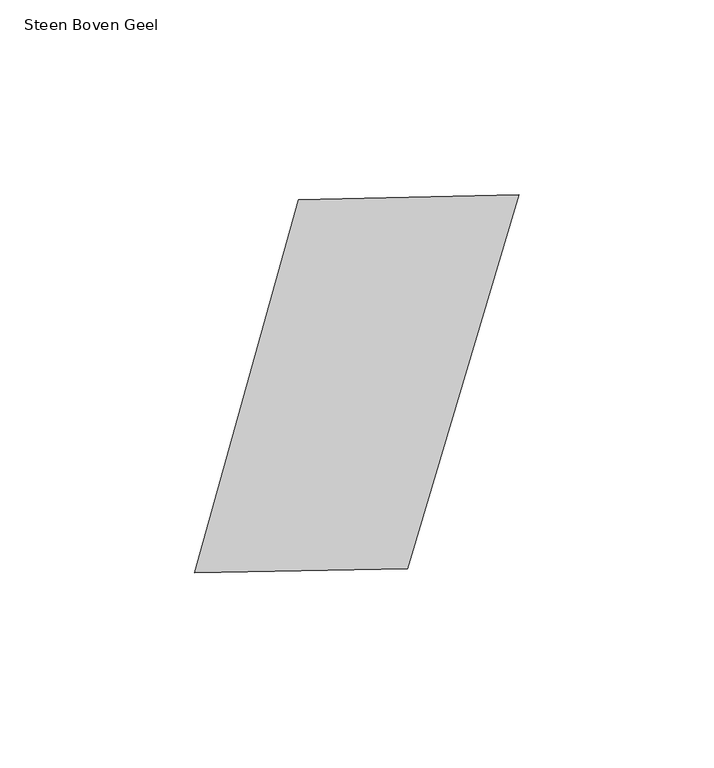
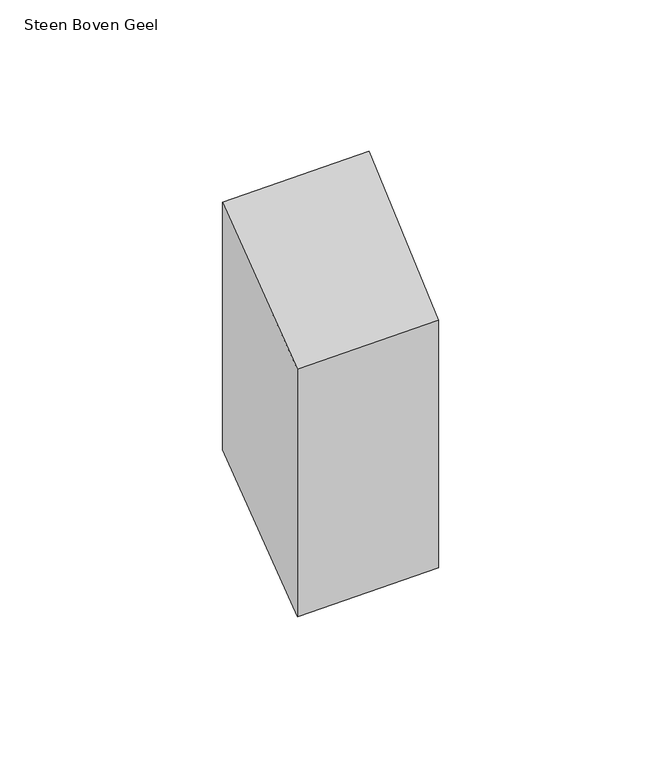
"""IFC4 building model written with IfcOpenShell, lengths in millimetres: proxy geometry, 00_GMA_steen_versie_4 : Steen Boven Geel."""

from ifc_helpers import new_model, si_unit, origin, origin_with_axes, place, context, project, spatial, polyline, outline, extrude, source, transform, mapped, element, save


def steen_boven_geel_aaecdfea(model_context):
    return source(origin(), model_context, "Body", "SweptSolid", [
        extrude(outline(polyline([(115.6222482, 118.81651), (86.9203145, 22.9603951), (32.3904012, 21.851807), (58.9678313, 117.6383065), (115.6222482, 118.81651)])), origin_with_axes(), (0.0, 0.0, 1.0), 100.0),
    ])


if __name__ == "__main__":
    model = new_model("IFC4")
    model_context = context("Model", 3, world=origin())
    ifc_project = project(units=[si_unit("LENGTHUNIT", "METRE", prefix="MILLI")], contexts=[model_context])
    site = spatial("IfcSite", under=ifc_project)
    building = spatial("IfcBuilding", under=site)
    placement = place(None, origin())
    steen_boven_geel_shape = steen_boven_geel_aaecdfea(model_context)
    element("IfcBuildingElementProxy", 1, Name="00_GMA_steen_versie_4 : Steen Boven Geel", ObjectType="00_GMA_steen_versie_4 : Steen Boven Geel", at=placement, inside=building, context=model_context, shape_type="MappedRepresentation", body=[
        mapped(steen_boven_geel_shape, transform((0.0, 0.0, 0.0), x_axis=(1.0, 0.0, 0.0), y_axis=(0.0, 1.0, 0.0), z_axis=(0.0, 0.0, 1.0))),
    ])
    save(model, "model.ifc")

# Revit data of these elements
# Type "00_GMA_steen_versie_4 : Steen Boven Geel"
#   StootVoegHalfBoven [instance default] = 5 mm
#   StootVoegHalf [instance default] = 5 mm
#   StootVoegBreedteOnder = 10 mm
#   StootVoegBreedteBoven = 10 mm
#   Steendikte = 100 mm
#   LintVoegOnderHalf = 5 mm
#   LintVoegOnder = 10 mm
#   LintVoegBovenHalf = 0 mm
#   LintVoegBoven = 0 mm
#   materiaal = 21_steen_geel
#   MateriaalVoeg = none
#   Default Elevation = 0
# Element 1 (IfcBuildingElementProxy, "00_GMA_steen_versie_4 : Steen Boven Geel")
#   Materials on its faces: "21_steen_geel"
# Materials
#   "21_steen_geel": class "Unassigned", colour RGB 202 202 0, transparency 0, Cost = 0
